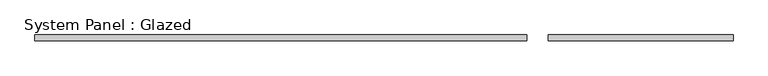
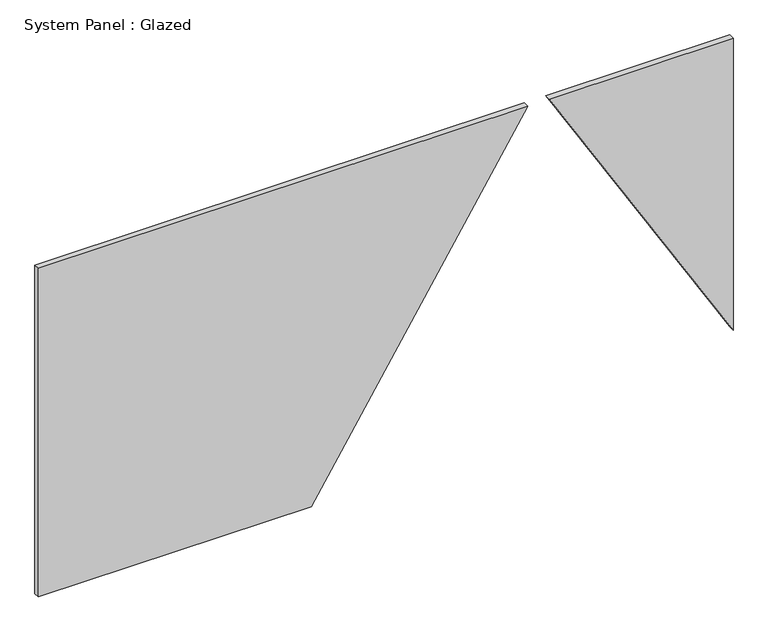
"""IFC4 building model written with IfcOpenShell, lengths in millimetres: plate geometry, System Panel : Glazed."""

from ifc_helpers import new_model, si_unit, frame, origin, place, context, project, spatial, polyline, outline, extrude, source, transform, mapped, element, save


def system_panel_glazed_440c1452(model_context):
    return source(origin(), model_context, "Body", "SweptSolid", [
        extrude(outline(polyline([(1500.0, 705.9127292), (167.838939, 1500.0), (1500.0, 1500.0), (1500.0, 705.9127292)])), frame((0.0, 24.5, 0.0), z_axis=(0.0, 1.0, 0.0), x_axis=(0.0, 0.0, 1.0)), (0.0, 0.0, 1.0), 25.0),
        extrude(outline(polyline([(0.0, -1500.0), (0.0, -321.0642638), (1500.0, 613.7086405), (1500.0, -1500.0), (0.0, -1500.0)])), frame((0.0, 24.5, 0.0), z_axis=(0.0, 1.0, 0.0), x_axis=(0.0, 0.0, 1.0)), (0.0, 0.0, 1.0), 25.0),
    ])


if __name__ == "__main__":
    model = new_model("IFC4")
    model_context = context("Model", 3, world=origin())
    ifc_project = project(units=[si_unit("LENGTHUNIT", "METRE", prefix="MILLI")], contexts=[model_context])
    site = spatial("IfcSite", under=ifc_project)
    building = spatial("IfcBuilding", under=site)
    placement = place(None, origin())
    system_panel_glazed_shape = system_panel_glazed_440c1452(model_context)
    element("IfcPlate", 1, ObjectType="System Panel : Glazed", at=placement, inside=building, context=model_context, shape_type="MappedRepresentation", body=[
        mapped(system_panel_glazed_shape, transform((0.0, 0.0, 0.0), x_axis=(1.0, 0.0, 0.0), y_axis=(0.0, 1.0, 0.0), z_axis=(0.0, 0.0, 1.0))),
    ])
    save(model, "model.ifc")

# Revit data of these elements
# Type "System Panel : Glazed"
#   Construction Type Id = "GSP4R"
#   Analytic Construction = "1/8 in Pilkington single glazing"
#   Visual Light Transmittance = 0.9
#   Solar Heat Gain Coefficient = 0.86
#   Heat Transfer Coefficient (U) = 6.7069 W/(m²·K)
#   Define Thermal Properties by = 1
# Element 1 (IfcPlate, "System Panel : Glazed")
#   Materials on its faces: "Glass"
# Materials
#   "Glass": class "Glass", colour RGB 0 128 192, transparency 0.9, Description = "Soda Lime Glass", Cost = 0
